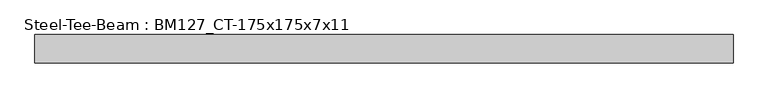
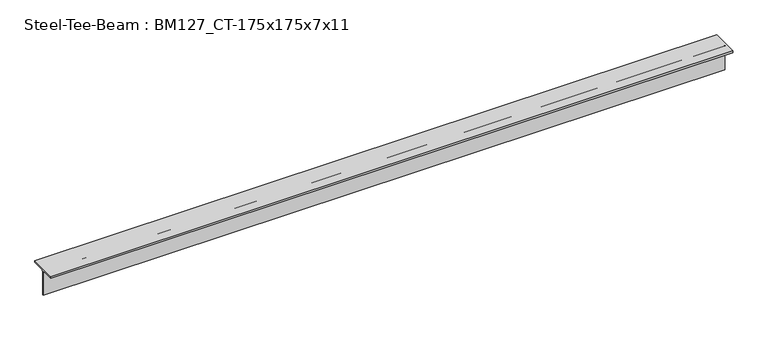
"""IFC4 building model written with IfcOpenShell, lengths in millimetres: beam geometry, Steel-Tee-Beam : BM127_CT-175x175x7x11."""

from ifc_helpers import new_model, si_unit, point, frame, frame_2d, origin, place, context, project, spatial, polyline, circle_curve, trimmed, segment, composite_curve, outline, extrude, source, transform, mapped, element, save


def steel_tee_beam_bm127_ct_175x175x7x11_5181b933(model_context):
    return source(origin(), model_context, "Body", "SweptSolid", [
        extrude(outline(composite_curve([segment(polyline([(87.5, 87.5), (87.5, 76.5), (17.5, 76.5)]), True, "CONTINUOUS"), segment(trimmed(circle_curve(frame_2d((17.5, 62.5)), 14.0), [point((17.5, 76.5))], [point((3.5, 62.5))], True, "CARTESIAN"), True, "CONTINUOUS"), segment(polyline([(3.5, 62.5), (3.5, -87.5), (-3.5, -87.5), (-3.5, 62.5)]), True, "CONTINUOUS"), segment(trimmed(circle_curve(frame_2d((-17.5, 62.5)), 14.0), [point((-3.5, 62.5))], [point((-17.5, 76.5))], True, "CARTESIAN"), True, "CONTINUOUS"), segment(polyline([(-17.5, 76.5), (-87.5, 76.5), (-87.5, 87.5), (87.5, 87.5)]), True, "CONTINUOUS")], self_intersect=False)), frame((-2106.825064, 0.0, 0.0), z_axis=(1.0, 0.0, 0.0), x_axis=(0.0, 1.0, 0.0)), (0.0, 0.0, 1.0), 4291.0318249),
    ])


if __name__ == "__main__":
    model = new_model("IFC4")
    model_context = context("Model", 3, world=origin())
    ifc_project = project(units=[si_unit("LENGTHUNIT", "METRE", prefix="MILLI")], contexts=[model_context])
    site = spatial("IfcSite", under=ifc_project)
    building = spatial("IfcBuilding", under=site)
    placement = place(None, origin())
    steel_tee_beam_bm127_ct_175x175x7x11_shape = steel_tee_beam_bm127_ct_175x175x7x11_5181b933(model_context)
    element("IfcBeam", 1, ObjectType="Steel-Tee-Beam : BM127_CT-175x175x7x11", at=placement, inside=building, context=model_context, shape_type="MappedRepresentation", body=[
        mapped(steel_tee_beam_bm127_ct_175x175x7x11_shape, transform((0.0, 0.0, 0.0), x_axis=(1.0, 0.0, 0.0), y_axis=(0.0, 1.0, 0.0), z_axis=(0.0, 0.0, 1.0))),
    ])
    save(model, "model.ifc")

# Revit data of these elements
# Type "Steel-Tee-Beam : BM127_CT-175x175x7x11"
#   Surface Area = 0.00 m²/m
#   Section Area = 31.57 cm²
#   Mass per Unit Length = 24.80 kg/m
#   Length [instance default] = 1524 mm
#   bf = 175 mm
#   d = 175 mm
#   k = 25 mm
#   kr = 14 mm
#   tf = 11 mm
#   tw = 7 mm
#   hec_material4 [instance default] = none
#   hec_material3 [instance default] = none
#   hec_material2 [instance default] = none
#   hec_material1 [instance default] = none
#   Structural Material [instance default] = Steel, 45-345
#   Assembly Code = ""
# Element 1 (IfcBeam, "Steel-Tee-Beam : BM127_CT-175x175x7x11")
#   hec_material3 = F01AC000-00002_Building/Shelter Fire Proofing Work_Intumescent Coating Type_1 hr. rating (UL 1709))
#   hec_material2 = S01AA010-00002_Main Steel Structure Fabrication Work_Shelter/Building_Steel Painting/Coating_for Fireproofed Steel Surface, Surface Preparation & Primer Coat
#   hec_material1 = S03AA029-00001_Main Steel Structure Erection Work_Shelter/Building_Light Steel
#   Structural Material = S01AA003-00001_Main Steel Structure Fabrication Work_Shelter/Building_Light Steel - Standard
#   Materials on its faces: "S01AA003-00001_Main Steel Structure Fabrication Work_Shelter/Building_Light Steel - Standard"
# Materials
#   "Steel, 45-345": class "Metal", colour RGB 189 187 185, transparency 0, Description = "Steel 345 MPa", Cost = 0
#   "S01AA003-00001_Main Steel Structure Fabrication Work_Shelter/Building_Light Steel - Standard": class "Metal", colour RGB 120 120 120, transparency 0, Comments = "(30KG/M>Weight)", Description = "Structural steel 50ksi", W00) Work Master Code = "S01AA003-00001", W01) Work Master_Lv1 = "Main Steel Structure Fabrication Work", W02) Work Master_Lv2 = "Shelter/Building", W03) Work Master_Spec.1 = "Light Steel - Standard (30KG/M>Weight)", Cost = 0
#   "F01AC000-00002_Building/Shelter Fire Proofing Work_Intumescent Coating Type_1 hr. rating (UL 1709))": class "Metal", colour RGB 255 128 128, transparency 0, Description = "Paint finished steel", W00) Work Master Code = "F01AC000-00002", W01) Work Master_Lv1 = "Building/Shelter Fire Proofing Work", W02) Work Master_Lv2 = "Intumescent Coating Type", W03) Work Master_Spec.1 = "1 hr. rating (UL 1709)", Cost = 0
#   "S01AA010-00002_Main Steel Structure Fabrication Work_Shelter/Building_Steel Painting/Coating_for Fireproofed Steel Surface, Surface Preparation & Primer Coat": class "Metal", colour RGB 120 120 120, transparency 0, Description = "Paint finished steel", W00) Work Master Code = "SS01AA010-00002", W01) Work Master_Lv1 = "Main Steel Structure Fabrication Work", W02) Work Master_Lv2 = "Shelter/Building", W03) Work Master_Spec.1 = "Steel Painting/Coating", W04) Work Master_Spec.2 = "for Fireproofed Steel Surface, Surface Preparation & Primer Coat", Cost = 0
#   "S03AA029-00001_Main Steel Structure Erection Work_Shelter/Building_Light Steel": class "Metal", colour RGB 120 120 120, transparency 0, Comments = "(30KG/M>Weight)", Description = "Structural steel 50ksi", W00) Work Master Code = "S03AA029-00001", W01) Work Master_Lv1 = "Main Steel Structure Erection Work", W02) Work Master_Lv2 = "Shelter/Building", W03) Work Master_Spec.1 = "Light Steel (30KG/M>Weight)", Cost = 0
